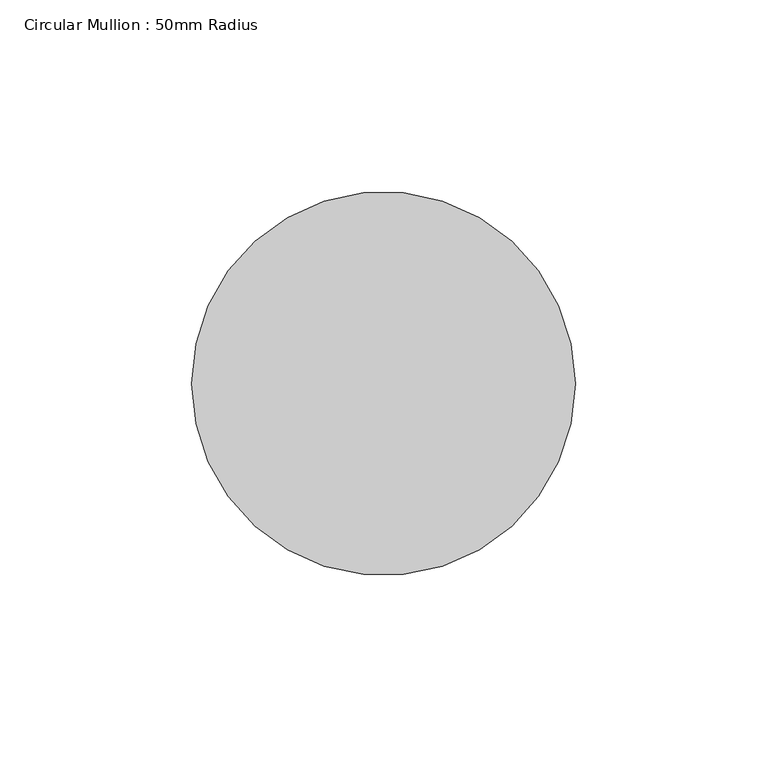
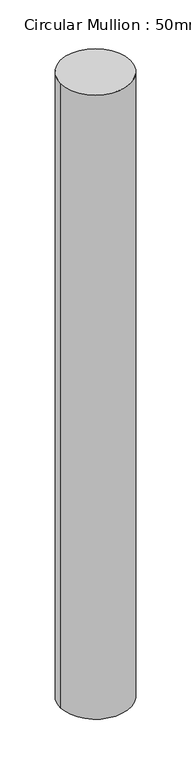
"""IFC4 building model written with IfcOpenShell, lengths in millimetres: member geometry, Circular Mullion : 50mm Radius."""

from ifc_helpers import new_model, si_unit, point, frame, origin, origin_2d, place, context, project, spatial, circle_curve, trimmed, segment, composite_curve, outline, extrude, source, transform, mapped, element, save


def circular_mullion_50mm_radius_b7ca167f(model_context):
    return source(origin(), model_context, "Body", "SweptSolid", [
        extrude(outline(composite_curve([segment(trimmed(circle_curve(origin_2d(), 50.0), [point((50.0, 0.0))], [point((-50.0, 0.0))], False, "CARTESIAN"), True, "CONTINUOUS"), segment(trimmed(circle_curve(origin_2d(), 50.0), [point((-50.0, 0.0))], [point((50.0, 0.0))], False, "CARTESIAN"), True, "CONTINUOUS")], self_intersect=False)), frame((0.0, 0.0, -944.7718579), z_axis=(0.0, 0.0, 1.0), x_axis=(1.0, 0.0, 0.0)), (0.0, 0.0, 1.0), 944.7718579),
    ])


if __name__ == "__main__":
    model = new_model("IFC4")
    model_context = context("Model", 3, world=origin())
    ifc_project = project(units=[si_unit("LENGTHUNIT", "METRE", prefix="MILLI")], contexts=[model_context])
    site = spatial("IfcSite", under=ifc_project)
    building = spatial("IfcBuilding", under=site)
    placement = place(None, origin())
    circular_mullion_50mm_radius_shape = circular_mullion_50mm_radius_b7ca167f(model_context)
    element("IfcMember", 1, ObjectType="Circular Mullion : 50mm Radius", at=placement, inside=building, context=model_context, shape_type="MappedRepresentation", body=[
        mapped(circular_mullion_50mm_radius_shape, transform((0.0, 0.0, 0.0), x_axis=(1.0, 0.0, 0.0), y_axis=(0.0, 1.0, 0.0), z_axis=(0.0, 0.0, 1.0))),
    ])
    save(model, "model.ifc")

# Revit data of these elements
# Type "Circular Mullion : 50mm Radius"
#   built-in parameter 1007350 = 0.164042 (stored number, unit not read)
# Element 1 (IfcMember, "Circular Mullion : 50mm Radius")
#   Materials on its faces: "Aluminium"
# Materials
#   "Aluminium": class "Metal", colour RGB 247 247 247, transparency 0, Description = "Aluminium 6061", Cost = 0
